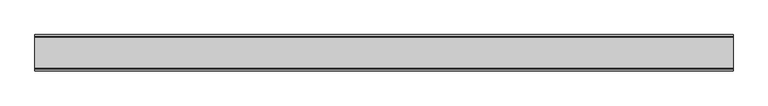
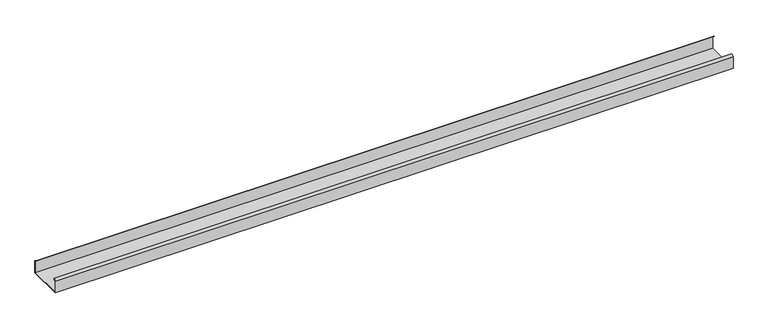
"""IFC4 building model written with IfcOpenShell, lengths in millimetres: proxy geometry, Generic Models 7:Generic Models 1:1:Generic Models 1:1 : Generic Models 7:Generic Models 1:337419:11 : Generic Models 7:Generic Models 1:1:Generic Models 1:1 : Generic Models 7:Generic Models 1:337419:306201."""

from ifc_helpers import new_model, si_unit, frame, origin, place, context, project, spatial, polyline, outline, extrude, source, transform, mapped, element, save


def generic_models_556c004d(model_context):
    return source(origin(), model_context, "Body", "SweptSolid", [
        extrude(outline(polyline([(-567932.6413841, 3675.0625), (-568186.6413841, 3675.0625), (-568186.6413841, 3763.9625), (-568172.0482375, 3776.207604), (-568170.2624931, 3774.0794367), (-568183.8632591, 3762.667039), (-568183.8632591, 3677.840625), (-567935.4195091, 3677.840625), (-567935.4195091, 3762.667039), (-567949.0202751, 3774.0794367), (-567947.2345307, 3776.207604), (-567932.6413841, 3763.9625), (-567932.6413841, 3675.0625)])), frame((591306.0367239, 0.0, 0.0), z_axis=(1.0, 0.0, 0.0), x_axis=(0.0, 1.0, 0.0)), (0.0, 0.0, 1.0), 4876.8),
    ])


if __name__ == "__main__":
    model = new_model("IFC4")
    model_context = context("Model", 3, world=origin())
    ifc_project = project(units=[si_unit("LENGTHUNIT", "METRE", prefix="MILLI")], contexts=[model_context])
    site = spatial("IfcSite", under=ifc_project)
    building = spatial("IfcBuilding", under=site)
    placement = place(None, origin())
    generic_models_shape = generic_models_556c004d(model_context)
    element("IfcBuildingElementProxy", 1, Name="Generic Models 7:Generic Models 1:1:Generic Models 1:1 : Generic Models 7:Generic Models 1:337419:11 : Generic Models 7:Generic Models 1:1:Generic Models 1:1 : Generic Models 7:Generic Models 1:337419:306201", ObjectType="Generic Models 7:Generic Models 1:1:Generic Models 1:1 : Generic Models 7:Generic Models 1:337419:11 : Generic Models 7:Generic Models 1:1:Generic Models 1:1 : Generic Models 7:Generic Models 1:337419:306201", at=placement, inside=building, context=model_context, shape_type="MappedRepresentation", body=[
        mapped(generic_models_shape, transform((0.0, 0.0, 0.0), x_axis=(1.0, 0.0, 0.0), y_axis=(0.0, 1.0, 0.0), z_axis=(0.0, 0.0, 1.0))),
    ])
    save(model, "model.ifc")

# Revit data of these elements
# Type "Generic Models 7:Generic Models 1:1:Generic Models 1:1 : Generic Models 7:Generic Models 1:337419:11 : Generic Models 7:Generic Models 1:1:Generic Models 1:1 : Generic Models 7:Generic Models 1:337419:306201"
#   NameOverride = "Generic Models 7:Generic Models 1:1:Generic Models 1:1 : Generic Models 7:Generic Models 1:337419:306201"
#   ObjectTypeOverride = "Generic Models 1:1 : Generic Models 7:Generic Models 1:337419"
#   Reference = "Generic Models 1"
#   Tag = "306201"
# Element 1 (IfcBuildingElementProxy, "Generic Models 7:Generic Models 1:1:Generic Models 1:1 : Generic Models 7:Generic Models 1:337419:11 : Generic Models 7:Generic Models 1:1:Generic Models 1:1 : Generic Models 7:Generic Models 1:337419:306201")
#   Materials on its faces: "'ZEE' SECTION (8.0x3.5Z - SEE STRUCT. DWGS)"
# Materials
#   "'ZEE' SECTION (8.0x3.5Z - SEE STRUCT. DWGS)": class "Unassigned", colour RGB 210 209 208, transparency 0, Keynote = "M05121300.02", Cost = 0
